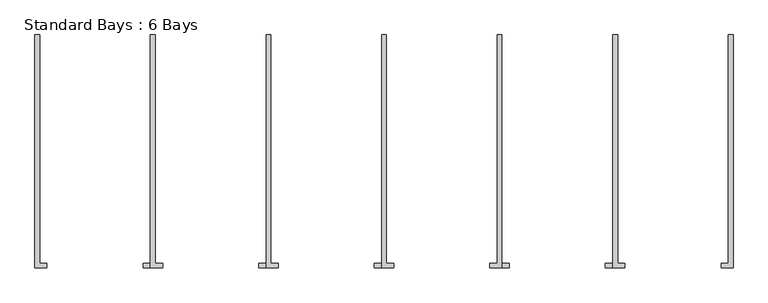
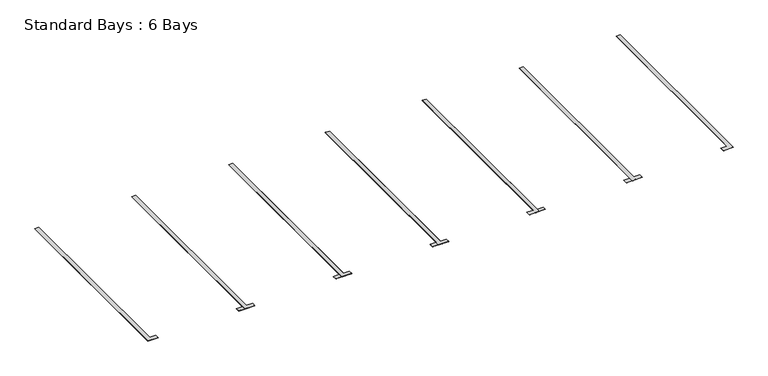
"""IFC4 building model written with IfcOpenShell, lengths in millimetres: proxy geometry, Standard Bays : 6 Bays."""

import ifcopenshell
import ifcopenshell.guid

model = None  # the IFC model being written
_history = None  # IfcOwnerHistory: only IFC2X3 demands one
_inside = {}  # id of a spatial element -> (the spatial element, [elements in it])
_under = {}  # id of a project, library or spatial element -> (it, [spatial elements below it])
_declared = {}  # id of a project -> (the project, [libraries it declares])
_typed = {}  # id of a type object -> (the type object, [elements of that type])
_made_of = {}  # id of a material, layer set ... -> (it, [elements and type objects made of it])


def new_model(schema):
    """Start an empty IFC model of exactly this schema.

    Asked for "IFC4X3", IfcOpenShell would pick the latest addendum, in which some entities
    have other attributes; the version numbers below select the first issue.
    IFC2X3 requires an IfcOwnerHistory on every rooted entity: one is made here for all.
    """
    global model, _history
    if schema == "IFC4X3":
        model = ifcopenshell.file(schema_version=(4, 3, 0, 0))
    else:
        model = ifcopenshell.file(schema=schema)
    _inside.clear()
    _under.clear()
    _declared.clear()
    _typed.clear()
    _made_of.clear()
    _history = None
    if model.schema == "IFC2X3":
        org = make("IfcOrganization", Name="unknown")
        user = make(
            "IfcPersonAndOrganization",
            ThePerson=make("IfcPerson", FamilyName="unknown"),
            TheOrganization=org,
        )
        app = make(
            "IfcApplication",
            ApplicationDeveloper=org,
            Version="unknown",
            ApplicationFullName="unknown",
            ApplicationIdentifier="unknown",
        )
        _history = make(
            "IfcOwnerHistory",
            OwningUser=user,
            OwningApplication=app,
            ChangeAction="ADDED",
            CreationDate=0,
        )
    return model


def make(cls, **values):
    """One entity of the class cls with the attributes given. An attribute that is None is left unset."""
    return model.create_entity(
        cls, **{name: value for name, value in values.items() if value is not None}
    )


def rooted(cls, **values):
    """An entity with a GlobalId (a new one), such as an element, a storey or a relation."""
    return make(cls, GlobalId=ifcopenshell.guid.new(), OwnerHistory=_history, **values)


def si_unit(unit_type, name, prefix=None):
    """IfcSIUnit, for example si_unit("LENGTHUNIT", "METRE", prefix="MILLI")."""
    return make("IfcSIUnit", UnitType=unit_type, Prefix=prefix, Name=name)


def assignment(units):
    """IfcUnitAssignment: the units of a project."""
    return None if units is None else make("IfcUnitAssignment", Units=units)


def point(xyz):
    """IfcCartesianPoint."""
    return None if xyz is None else make("IfcCartesianPoint", Coordinates=xyz)


def direction(xyz):
    """IfcDirection."""
    return None if xyz is None else make("IfcDirection", DirectionRatios=xyz)


def frame(location, z_axis=None, x_axis=None):
    """IfcAxis2Placement3D, a coordinate frame: its origin and axes. An axis left out is left unset."""
    return make(
        "IfcAxis2Placement3D",
        Location=point(location),
        Axis=direction(z_axis),
        RefDirection=direction(x_axis),
    )


def origin():
    """The frame at (0, 0, 0) with its axes left unset."""
    return frame((0.0, 0.0, 0.0))


def origin_with_axes():
    """The frame at (0, 0, 0) with the z axis (0, 0, 1) and the x axis (1, 0, 0) written out."""
    return frame((0.0, 0.0, 0.0), z_axis=(0.0, 0.0, 1.0), x_axis=(1.0, 0.0, 0.0))


def place(relative_to, where):
    """IfcLocalPlacement: puts the frame where relative to a parent placement (None: the world)."""
    return make(
        "IfcLocalPlacement", PlacementRelTo=relative_to, RelativePlacement=where
    )


def context(
    kind, dimensions, precision=None, world=None, true_north=None, identifier=None
):
    """IfcGeometricRepresentationContext, for example the 3D "Model" context."""
    return make(
        "IfcGeometricRepresentationContext",
        ContextIdentifier=identifier,
        ContextType=kind,
        CoordinateSpaceDimension=dimensions,
        Precision=precision,
        WorldCoordinateSystem=world,
        TrueNorth=true_north,
    )


def project(units=None, contexts=None):
    """IfcProject with its units and contexts."""
    return rooted(
        "IfcProject",
        Name="project",
        RepresentationContexts=contexts,
        UnitsInContext=assignment(units),
    )


def spatial(cls, under=None, at=None, **own):
    """A site, building, storey or space (cls), placed at a placement, below another one or the project."""
    s = rooted(cls, ObjectPlacement=at, **own)
    if under is not None:
        _under.setdefault(under.id(), (under, []))[1].append(s)
    return s


def polyline(points):
    """IfcPolyline through the points."""
    return make("IfcPolyline", Points=[point(p) for p in points])


def outline(outer, holes=None, kind="AREA"):
    """IfcArbitraryClosedProfileDef: a profile drawn as a closed curve; with holes, ...WithVoids."""
    if holes is None:
        return make("IfcArbitraryClosedProfileDef", ProfileType=kind, OuterCurve=outer)
    return make(
        "IfcArbitraryProfileDefWithVoids",
        ProfileType=kind,
        OuterCurve=outer,
        InnerCurves=holes,
    )


def extrude(swept, where, along, depth):
    """IfcExtrudedAreaSolid: the profile swept, set in the frame where, extruded along a direction by depth."""
    return make(
        "IfcExtrudedAreaSolid",
        SweptArea=swept,
        Position=where,
        ExtrudedDirection=direction(along),
        Depth=depth,
    )


def shape(context_of_items, identifier, shape_type, items):
    """IfcShapeRepresentation: the items that make up one representation, for example the "Body"."""
    return make(
        "IfcShapeRepresentation",
        ContextOfItems=context_of_items,
        RepresentationIdentifier=identifier,
        RepresentationType=shape_type,
        Items=items,
    )


def source(mapping_origin, context_of_items, identifier, shape_type, items):
    """IfcRepresentationMap: a shape defined once, which mapped items show again and again."""
    return make(
        "IfcRepresentationMap",
        MappingOrigin=mapping_origin,
        MappedRepresentation=shape(context_of_items, identifier, shape_type, items),
    )


def transform(
    local_origin,
    x_axis=None,
    y_axis=None,
    z_axis=None,
    scale=None,
    scale2=None,
    scale3=None,
    uniform=True,
):
    """IfcCartesianTransformationOperator3D, or its non-uniform kind. x_axis, y_axis, z_axis: its Axis1, 2, 3."""
    if uniform:
        return make(
            "IfcCartesianTransformationOperator3D",
            Axis1=direction(x_axis),
            Axis2=direction(y_axis),
            LocalOrigin=point(local_origin),
            Scale=scale,
            Axis3=direction(z_axis),
        )
    return make(
        "IfcCartesianTransformationOperator3DnonUniform",
        Axis1=direction(x_axis),
        Axis2=direction(y_axis),
        LocalOrigin=point(local_origin),
        Scale=scale,
        Axis3=direction(z_axis),
        Scale2=scale2,
        Scale3=scale3,
    )


def mapped(mapping_source, mapping_target):
    """IfcMappedItem: shows the shape of a source again, moved by a transform."""
    return make(
        "IfcMappedItem", MappingSource=mapping_source, MappingTarget=mapping_target
    )


def made_of(thing, what):
    """Note that an element or type object is made of a material, layer set ...; save() writes the relation."""
    if what is not None:
        _made_of.setdefault(what.id(), (what, []))[1].append(thing)
    return thing


def element(
    cls,
    number,
    at=None,
    inside=None,
    cuts=None,
    type_object=None,
    material=None,
    context=None,
    identifier="Body",
    shape_type=None,
    held_by="IfcProductDefinitionShape",
    body=None,
    shapes=None,
    **own,
):
    """One element of the class cls, such as IfcWall. Its Tag is "e" and its number.

    at: its placement. inside: the storey or other place that contains it. cuts: it is an
    opening in that element (IfcRelVoidsElement). A single representation is given by context,
    identifier, shape_type and body (its items); several are given by shapes. held_by: the class
    of the entity that holds the representations. save() writes the other relations.
    """
    e = rooted(cls, Tag="e%d" % number, ObjectPlacement=at, **own)
    if body is not None:
        shapes = [shape(context, identifier, shape_type, body)]
    if shapes is not None:
        e.Representation = make(held_by, Representations=shapes)
    if inside is not None:
        _inside.setdefault(inside.id(), (inside, []))[1].append(e)
    if cuts is not None:
        rooted(
            "IfcRelVoidsElement", RelatingBuildingElement=cuts, RelatedOpeningElement=e
        )
    if type_object is not None:
        _typed.setdefault(type_object.id(), (type_object, []))[1].append(e)
    return made_of(e, material)


def aggregate(whole, parts):
    """IfcRelAggregates: a whole, such as a stair, and the parts it consists of."""
    return rooted("IfcRelAggregates", RelatingObject=whole, RelatedObjects=parts)


def save(model, path):
    """Write the relations noted so far, then the file.

    IfcRelAggregates (storeys below a building ...), IfcRelContainedInSpatialStructure (elements
    in a storey), IfcRelDefinesByType, IfcRelAssociatesMaterial and IfcRelDeclares: one each for
    every whole, place, type object, material and project.
    """
    for whole, parts in _under.values():
        aggregate(whole, parts)
    for where, things in _inside.values():
        rooted(
            "IfcRelContainedInSpatialStructure",
            RelatedElements=things,
            RelatingStructure=where,
        )
    for kind, things in _typed.values():
        rooted("IfcRelDefinesByType", RelatedObjects=things, RelatingType=kind)
    for what, things in _made_of.values():
        rooted("IfcRelAssociatesMaterial", RelatedObjects=things, RelatingMaterial=what)
    for by, libraries in _declared.values():
        rooted("IfcRelDeclares", RelatingContext=by, RelatedDefinitions=libraries)
    model.write(path)


def standard_bays_6_bays_a1d699d5(model_context):
    return source(origin(), model_context, "Body", "SweptSolid", [
        extrude(outline(polyline([(14350.0, 0.0), (14450.0, 0.0), (14450.0, -4850.0), (14200.0, -4850.0), (14200.0, -4750.0), (14350.0, -4750.0), (14350.0, 0.0)])), origin_with_axes(), (0.0, 0.0, 1.0), 3.175),
        extrude(outline(polyline([(11950.0, 0.0), (12050.0, 0.0), (12050.0, -4750.0), (12200.0, -4750.0), (12200.0, -4850.0), (11950.0, -4850.0), (11950.0, 0.0)])), origin_with_axes(), (0.0, 0.0, 1.0), 3.175),
        extrude(outline(polyline([(9550.0, 0.0), (9650.0, 0.0), (9650.0, -4850.0), (9400.0, -4850.0), (9400.0, -4750.0), (9550.0, -4750.0), (9550.0, 0.0)])), origin_with_axes(), (0.0, 0.0, 1.0), 3.175),
        extrude(outline(polyline([(7150.0, 0.0), (7250.0, 0.0), (7250.0, -4750.0), (7400.0, -4750.0), (7400.0, -4850.0), (7150.0, -4850.0), (7150.0, 0.0)])), origin_with_axes(), (0.0, 0.0, 1.0), 3.175),
        extrude(outline(polyline([(7150.0, 0.0), (7250.0, 0.0), (7250.0, -4850.0), (7000.0, -4850.0), (7000.0, -4750.0), (7150.0, -4750.0), (7150.0, 0.0)])), origin_with_axes(), (0.0, 0.0, 1.0), 3.175),
        extrude(outline(polyline([(4750.0, 0.0), (4850.0, 0.0), (4850.0, -4750.0), (5000.0, -4750.0), (5000.0, -4850.0), (4750.0, -4850.0), (4750.0, 0.0)])), origin_with_axes(), (0.0, 0.0, 1.0), 3.175),
        extrude(outline(polyline([(4750.0, 0.0), (4850.0, 0.0), (4850.0, -4850.0), (4600.0, -4850.0), (4600.0, -4750.0), (4750.0, -4750.0), (4750.0, 0.0)])), origin_with_axes(), (0.0, 0.0, 1.0), 3.175),
        extrude(outline(polyline([(2350.0, 0.0), (2450.0, 0.0), (2450.0, -4750.0), (2600.0, -4750.0), (2600.0, -4850.0), (2350.0, -4850.0), (2350.0, 0.0)])), origin_with_axes(), (0.0, 0.0, 1.0), 3.175),
        extrude(outline(polyline([(11950.0, 0.0), (12050.0, 0.0), (12050.0, -4850.0), (11800.0, -4850.0), (11800.0, -4750.0), (11950.0, -4750.0), (11950.0, 0.0)])), origin_with_axes(), (0.0, 0.0, 1.0), 3.175),
        extrude(outline(polyline([(9550.0, 0.0), (9650.0, 0.0), (9650.0, -4750.0), (9800.0, -4750.0), (9800.0, -4850.0), (9550.0, -4850.0), (9550.0, 0.0)])), origin_with_axes(), (0.0, 0.0, 1.0), 3.175),
        extrude(outline(polyline([(2350.0, 0.0), (2450.0, 0.0), (2450.0, -4850.0), (2200.0, -4850.0), (2200.0, -4750.0), (2350.0, -4750.0), (2350.0, 0.0)])), origin_with_axes(), (0.0, 0.0, 1.0), 3.175),
        extrude(outline(polyline([(-50.0, 0.0), (50.0, 0.0), (50.0, -4750.0), (200.0, -4750.0), (200.0, -4850.0), (-50.0, -4850.0), (-50.0, 0.0)])), origin_with_axes(), (0.0, 0.0, 1.0), 3.175),
    ])


if __name__ == "__main__":
    model = new_model("IFC4")
    model_context = context("Model", 3, world=origin())
    ifc_project = project(units=[si_unit("LENGTHUNIT", "METRE", prefix="MILLI")], contexts=[model_context])
    site = spatial("IfcSite", under=ifc_project)
    building = spatial("IfcBuilding", under=site)
    placement = place(None, origin())
    standard_bays_6_bays_shape = standard_bays_6_bays_a1d699d5(model_context)
    element("IfcBuildingElementProxy", 1, Name="Standard Bays : 6 Bays", ObjectType="Standard Bays : 6 Bays", at=placement, inside=building, context=model_context, shape_type="MappedRepresentation", body=[
        mapped(standard_bays_6_bays_shape, transform((0.0, 0.0, 0.0), x_axis=(1.0, 0.0, 0.0), y_axis=(0.0, 1.0, 0.0), z_axis=(0.0, 0.0, 1.0))),
    ])
    save(model, "model.ifc")

# Revit data of these elements
# Type "Standard Bays : 6 Bays"
#   Keynote = "Q22/185"
#   Length [instance default] = 14400 mm
#   Bay Width = 2400 mm
#   Bay Length = 4800 mm
#   No of Bays in Array [instance default] = 5
#   No of Bays [instance default] = 6
#   Material - White Lining = Paint - White Lining
# Element 1 (IfcBuildingElementProxy, "Standard Bays : 6 Bays")
#   Materials on its faces: "Paint - White Lining"
# Materials
#   "Paint - White Lining": class "Paint", colour RGB 239 247 247, transparency 0
